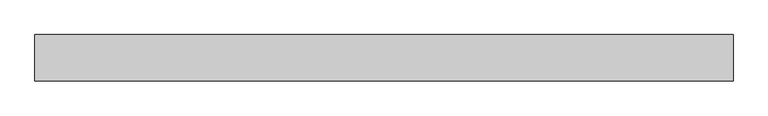
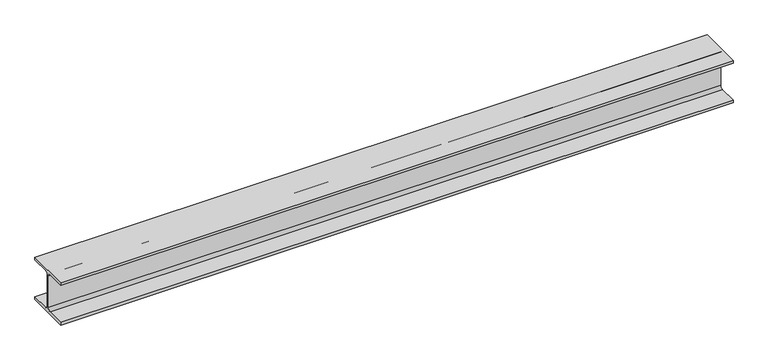
"""IFC4 building model written with IfcOpenShell, lengths in millimetres: beam geometry, 0912_Steel Framing_H-KSD3502 : H_SB_ASB_H-200x200x8x12."""

import ifcopenshell
import ifcopenshell.guid

model = None  # the IFC model being written
_history = None  # IfcOwnerHistory: only IFC2X3 demands one
_inside = {}  # id of a spatial element -> (the spatial element, [elements in it])
_under = {}  # id of a project, library or spatial element -> (it, [spatial elements below it])
_declared = {}  # id of a project -> (the project, [libraries it declares])
_typed = {}  # id of a type object -> (the type object, [elements of that type])
_made_of = {}  # id of a material, layer set ... -> (it, [elements and type objects made of it])


def new_model(schema):
    """Start an empty IFC model of exactly this schema.

    Asked for "IFC4X3", IfcOpenShell would pick the latest addendum, in which some entities
    have other attributes; the version numbers below select the first issue.
    IFC2X3 requires an IfcOwnerHistory on every rooted entity: one is made here for all.
    """
    global model, _history
    if schema == "IFC4X3":
        model = ifcopenshell.file(schema_version=(4, 3, 0, 0))
    else:
        model = ifcopenshell.file(schema=schema)
    _inside.clear()
    _under.clear()
    _declared.clear()
    _typed.clear()
    _made_of.clear()
    _history = None
    if model.schema == "IFC2X3":
        org = make("IfcOrganization", Name="unknown")
        user = make(
            "IfcPersonAndOrganization",
            ThePerson=make("IfcPerson", FamilyName="unknown"),
            TheOrganization=org,
        )
        app = make(
            "IfcApplication",
            ApplicationDeveloper=org,
            Version="unknown",
            ApplicationFullName="unknown",
            ApplicationIdentifier="unknown",
        )
        _history = make(
            "IfcOwnerHistory",
            OwningUser=user,
            OwningApplication=app,
            ChangeAction="ADDED",
            CreationDate=0,
        )
    return model


def make(cls, **values):
    """One entity of the class cls with the attributes given. An attribute that is None is left unset."""
    return model.create_entity(
        cls, **{name: value for name, value in values.items() if value is not None}
    )


def rooted(cls, **values):
    """An entity with a GlobalId (a new one), such as an element, a storey or a relation."""
    return make(cls, GlobalId=ifcopenshell.guid.new(), OwnerHistory=_history, **values)


def si_unit(unit_type, name, prefix=None):
    """IfcSIUnit, for example si_unit("LENGTHUNIT", "METRE", prefix="MILLI")."""
    return make("IfcSIUnit", UnitType=unit_type, Prefix=prefix, Name=name)


def assignment(units):
    """IfcUnitAssignment: the units of a project."""
    return None if units is None else make("IfcUnitAssignment", Units=units)


def point(xyz):
    """IfcCartesianPoint."""
    return None if xyz is None else make("IfcCartesianPoint", Coordinates=xyz)


def direction(xyz):
    """IfcDirection."""
    return None if xyz is None else make("IfcDirection", DirectionRatios=xyz)


def frame(location, z_axis=None, x_axis=None):
    """IfcAxis2Placement3D, a coordinate frame: its origin and axes. An axis left out is left unset."""
    return make(
        "IfcAxis2Placement3D",
        Location=point(location),
        Axis=direction(z_axis),
        RefDirection=direction(x_axis),
    )


def frame_2d(location, x_axis=None):
    """IfcAxis2Placement2D, a coordinate frame in the plane: its origin and x axis."""
    return make(
        "IfcAxis2Placement2D", Location=point(location), RefDirection=direction(x_axis)
    )


def origin():
    """The frame at (0, 0, 0) with its axes left unset."""
    return frame((0.0, 0.0, 0.0))


def place(relative_to, where):
    """IfcLocalPlacement: puts the frame where relative to a parent placement (None: the world)."""
    return make(
        "IfcLocalPlacement", PlacementRelTo=relative_to, RelativePlacement=where
    )


def context(
    kind, dimensions, precision=None, world=None, true_north=None, identifier=None
):
    """IfcGeometricRepresentationContext, for example the 3D "Model" context."""
    return make(
        "IfcGeometricRepresentationContext",
        ContextIdentifier=identifier,
        ContextType=kind,
        CoordinateSpaceDimension=dimensions,
        Precision=precision,
        WorldCoordinateSystem=world,
        TrueNorth=true_north,
    )


def project(units=None, contexts=None):
    """IfcProject with its units and contexts."""
    return rooted(
        "IfcProject",
        Name="project",
        RepresentationContexts=contexts,
        UnitsInContext=assignment(units),
    )


def spatial(cls, under=None, at=None, **own):
    """A site, building, storey or space (cls), placed at a placement, below another one or the project."""
    s = rooted(cls, ObjectPlacement=at, **own)
    if under is not None:
        _under.setdefault(under.id(), (under, []))[1].append(s)
    return s


def polyline(points):
    """IfcPolyline through the points."""
    return make("IfcPolyline", Points=[point(p) for p in points])


def circle_curve(where, radius):
    """IfcCircle in the frame where."""
    return make("IfcCircle", Position=where, Radius=radius)


def trimmed(basis, trim1, trim2, sense, master):
    """IfcTrimmedCurve: the piece of a basis curve between two trims."""
    return make(
        "IfcTrimmedCurve",
        BasisCurve=basis,
        Trim1=trim1,
        Trim2=trim2,
        SenseAgreement=sense,
        MasterRepresentation=master,
    )


def segment(curve, same_sense, transition):
    """IfcCompositeCurveSegment."""
    return make(
        "IfcCompositeCurveSegment",
        Transition=transition,
        SameSense=same_sense,
        ParentCurve=curve,
    )


def composite_curve(segments, self_intersect=None):
    """IfcCompositeCurve: segments joined end to end."""
    return make("IfcCompositeCurve", Segments=segments, SelfIntersect=self_intersect)


def outline(outer, holes=None, kind="AREA"):
    """IfcArbitraryClosedProfileDef: a profile drawn as a closed curve; with holes, ...WithVoids."""
    if holes is None:
        return make("IfcArbitraryClosedProfileDef", ProfileType=kind, OuterCurve=outer)
    return make(
        "IfcArbitraryProfileDefWithVoids",
        ProfileType=kind,
        OuterCurve=outer,
        InnerCurves=holes,
    )


def extrude(swept, where, along, depth):
    """IfcExtrudedAreaSolid: the profile swept, set in the frame where, extruded along a direction by depth."""
    return make(
        "IfcExtrudedAreaSolid",
        SweptArea=swept,
        Position=where,
        ExtrudedDirection=direction(along),
        Depth=depth,
    )


def shape(context_of_items, identifier, shape_type, items):
    """IfcShapeRepresentation: the items that make up one representation, for example the "Body"."""
    return make(
        "IfcShapeRepresentation",
        ContextOfItems=context_of_items,
        RepresentationIdentifier=identifier,
        RepresentationType=shape_type,
        Items=items,
    )


def source(mapping_origin, context_of_items, identifier, shape_type, items):
    """IfcRepresentationMap: a shape defined once, which mapped items show again and again."""
    return make(
        "IfcRepresentationMap",
        MappingOrigin=mapping_origin,
        MappedRepresentation=shape(context_of_items, identifier, shape_type, items),
    )


def transform(
    local_origin,
    x_axis=None,
    y_axis=None,
    z_axis=None,
    scale=None,
    scale2=None,
    scale3=None,
    uniform=True,
):
    """IfcCartesianTransformationOperator3D, or its non-uniform kind. x_axis, y_axis, z_axis: its Axis1, 2, 3."""
    if uniform:
        return make(
            "IfcCartesianTransformationOperator3D",
            Axis1=direction(x_axis),
            Axis2=direction(y_axis),
            LocalOrigin=point(local_origin),
            Scale=scale,
            Axis3=direction(z_axis),
        )
    return make(
        "IfcCartesianTransformationOperator3DnonUniform",
        Axis1=direction(x_axis),
        Axis2=direction(y_axis),
        LocalOrigin=point(local_origin),
        Scale=scale,
        Axis3=direction(z_axis),
        Scale2=scale2,
        Scale3=scale3,
    )


def mapped(mapping_source, mapping_target):
    """IfcMappedItem: shows the shape of a source again, moved by a transform."""
    return make(
        "IfcMappedItem", MappingSource=mapping_source, MappingTarget=mapping_target
    )


def made_of(thing, what):
    """Note that an element or type object is made of a material, layer set ...; save() writes the relation."""
    if what is not None:
        _made_of.setdefault(what.id(), (what, []))[1].append(thing)
    return thing


def element(
    cls,
    number,
    at=None,
    inside=None,
    cuts=None,
    type_object=None,
    material=None,
    context=None,
    identifier="Body",
    shape_type=None,
    held_by="IfcProductDefinitionShape",
    body=None,
    shapes=None,
    **own,
):
    """One element of the class cls, such as IfcWall. Its Tag is "e" and its number.

    at: its placement. inside: the storey or other place that contains it. cuts: it is an
    opening in that element (IfcRelVoidsElement). A single representation is given by context,
    identifier, shape_type and body (its items); several are given by shapes. held_by: the class
    of the entity that holds the representations. save() writes the other relations.
    """
    e = rooted(cls, Tag="e%d" % number, ObjectPlacement=at, **own)
    if body is not None:
        shapes = [shape(context, identifier, shape_type, body)]
    if shapes is not None:
        e.Representation = make(held_by, Representations=shapes)
    if inside is not None:
        _inside.setdefault(inside.id(), (inside, []))[1].append(e)
    if cuts is not None:
        rooted(
            "IfcRelVoidsElement", RelatingBuildingElement=cuts, RelatedOpeningElement=e
        )
    if type_object is not None:
        _typed.setdefault(type_object.id(), (type_object, []))[1].append(e)
    return made_of(e, material)


def aggregate(whole, parts):
    """IfcRelAggregates: a whole, such as a stair, and the parts it consists of."""
    return rooted("IfcRelAggregates", RelatingObject=whole, RelatedObjects=parts)


def save(model, path):
    """Write the relations noted so far, then the file.

    IfcRelAggregates (storeys below a building ...), IfcRelContainedInSpatialStructure (elements
    in a storey), IfcRelDefinesByType, IfcRelAssociatesMaterial and IfcRelDeclares: one each for
    every whole, place, type object, material and project.
    """
    for whole, parts in _under.values():
        aggregate(whole, parts)
    for where, things in _inside.values():
        rooted(
            "IfcRelContainedInSpatialStructure",
            RelatedElements=things,
            RelatingStructure=where,
        )
    for kind, things in _typed.values():
        rooted("IfcRelDefinesByType", RelatedObjects=things, RelatingType=kind)
    for what, things in _made_of.values():
        rooted("IfcRelAssociatesMaterial", RelatedObjects=things, RelatingMaterial=what)
    for by, libraries in _declared.values():
        rooted("IfcRelDeclares", RelatingContext=by, RelatedDefinitions=libraries)
    model.write(path)


def beam_3227815b(model_context):
    return source(origin(), model_context, "Body", "SweptSolid", [
        extrude(outline(composite_curve([segment(polyline([(100.0, -88.0), (100.0, -100.0), (-100.0, -100.0), (-100.0, -88.0), (-17.0, -88.0)]), True, "CONTINUOUS"), segment(trimmed(circle_curve(frame_2d((-17.0, -75.0)), 13.0), [point((-17.0, -88.0))], [point((-4.0, -75.0))], True, "CARTESIAN"), True, "CONTINUOUS"), segment(polyline([(-4.0, -75.0), (-4.0, 75.0)]), True, "CONTINUOUS"), segment(trimmed(circle_curve(frame_2d((-17.0, 75.0)), 13.0), [point((-4.0, 75.0))], [point((-17.0, 88.0))], True, "CARTESIAN"), True, "CONTINUOUS"), segment(polyline([(-17.0, 88.0), (-100.0, 88.0), (-100.0, 100.0), (100.0, 100.0), (100.0, 88.0), (17.0, 88.0)]), True, "CONTINUOUS"), segment(trimmed(circle_curve(frame_2d((17.0, 75.0)), 13.0), [point((17.0, 88.0))], [point((4.0, 75.0))], True, "CARTESIAN"), True, "CONTINUOUS"), segment(polyline([(4.0, 75.0), (4.0, -75.0)]), True, "CONTINUOUS"), segment(trimmed(circle_curve(frame_2d((17.0, -75.0)), 13.0), [point((4.0, -75.0))], [point((17.0, -88.0))], True, "CARTESIAN"), True, "CONTINUOUS"), segment(polyline([(17.0, -88.0), (100.0, -88.0)]), True, "CONTINUOUS")], self_intersect=False)), frame((-1321.0203679, 0.0, 0.0), z_axis=(1.0, 0.0, 0.0), x_axis=(0.0, 1.0, 0.0)), (0.0, 0.0, 1.0), 3005.8055003),
    ])


if __name__ == "__main__":
    model = new_model("IFC4")
    model_context = context("Model", 3, world=origin())
    ifc_project = project(units=[si_unit("LENGTHUNIT", "METRE", prefix="MILLI")], contexts=[model_context])
    site = spatial("IfcSite", under=ifc_project)
    building = spatial("IfcBuilding", under=site)
    placement = place(None, origin())
    beam_shape = beam_3227815b(model_context)
    element("IfcBeam", 1, ObjectType="0912_Steel Framing_H-KSD3502 : H_SB_ASB_H-200x200x8x12", at=placement, inside=building, context=model_context, shape_type="MappedRepresentation", body=[
        mapped(beam_shape, transform((0.0, 0.0, 0.0), x_axis=(1.0, 0.0, 0.0), y_axis=(0.0, 1.0, 0.0), z_axis=(0.0, 0.0, 1.0))),
    ])
    save(model, "model.ifc")

# Revit data of these elements
# Type "0912_Steel Framing_H-KSD3502 : H_SB_ASB_H-200x200x8x12"
#   H_WM Code_1 = "S01AA002-00001 | Main Steel Structure Fabrication Work | Shelter/Building | Medium Steel - Standard (90KG/M>Weight≥30KG/M) | Material: (   )"
#   H_WM Code_2 = "S03AA028-00001 | Main Steel Structure Erection Work | Shelter/Building | Medium Steel (90KG/M>Weight≥30KG/M) | Material: (   )"
#   H_WM Code_3 = "S01AA010-00001 | Main Steel Structure Fabrication Work | Shelter/Building | Steel Painting/Coating | for Non-Fireproofed Steel Surface, Surface Preparation, Primer, Second & Final Coat | Material: (   )"
#   H_Q'ty Cal Type Tag = "SB-Q2"
#   Width = 20.0 cm
#   Web Thickness = 0.8 cm
#   Web Fillet = 1.3 cm
#   Warping Constant = 141000.0 cm⁶
#   W = 0
#   Torsional Moment of Inertia = 26.2485 cm⁴
#   Section Area = 63.53 cm²
#   Plastic Modulus weak axis = 244.0 cm³
#   Plastic Modulus strong axis = 525.0 cm³
#   Perimeter = 1.16 m²/m
#   Nominal Weight = 49.90 kgf/m
#   Moment of Inertia weak axis = 1600.00 cm⁴
#   Moment of Inertia strong axis = 4720.00 cm⁴
#   Height = 20.0 cm
#   Flange Thickness = 1.2 cm
#   Elastic Modulus weak axis = 160.0 cm³
#   Elastic Modulus strong axis = 472.0 cm³
#   Centroid Vertical = 10.0 cm
#   Centroid Horizontal = 10.0 cm
#   Ix = 47200000
#   Length [instance default] = 1.5240 m
#   Zx = 525000
#   b = 0.2000 m
#   h = 0.2000 m
#   r = 0.0130 m
#   s = 0.0080 m
#   t = 0.0120 m
#   A = 0.006353 m²
#   Structural Material [instance default] = Steel, 45-345
#   Assembly Code = ""
# Element 1 (IfcBeam, "0912_Steel Framing_H-KSD3502 : H_SB_ASB_H-200x200x8x12")
#   Structural Material = none
# Materials
#   "Steel, 45-345": class "Metal", colour RGB 189 187 185, transparency 0, Description = "Steel 345 MPa", Cost = 0
